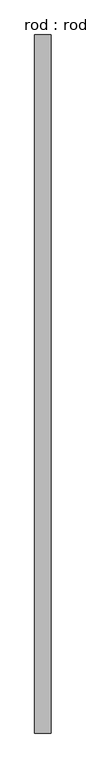
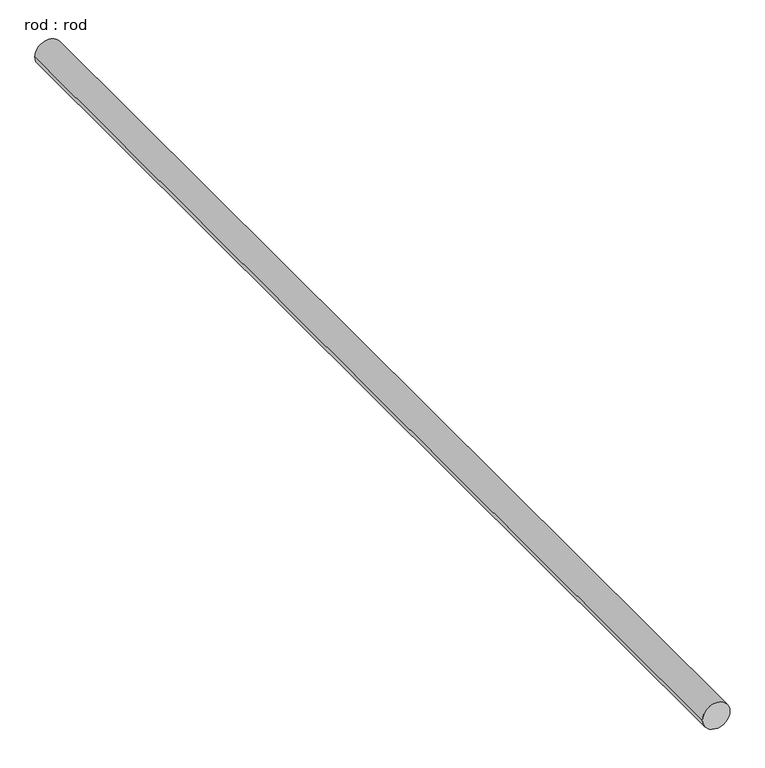
"""IFC4 building model written with IfcOpenShell, lengths in millimetres: proxy geometry, rod : rod."""

from ifc_helpers import new_model, si_unit, point, frame, frame_2d, origin, place, context, project, spatial, circle_curve, trimmed, segment, composite_curve, outline, extrude, source, transform, mapped, element, save


def rod_rod_0cf6e89c(model_context):
    return source(origin(), model_context, "Body", "SweptSolid", [
        extrude(outline(composite_curve([segment(trimmed(circle_curve(frame_2d((0.0108462, 0.0)), 200.0), [point((0.0108462, 200.0))], [point((0.0108462, -200.0))], False, "CARTESIAN"), True, "CONTINUOUS"), segment(trimmed(circle_curve(frame_2d((0.0108462, 0.0)), 200.0), [point((0.0108462, -200.0))], [point((0.0108462, 200.0))], False, "CARTESIAN"), True, "CONTINUOUS")], self_intersect=False)), frame((0.0, -4349.5154804, 0.0), z_axis=(0.0, 1.0, 0.0), x_axis=(0.0, 0.0, 1.0)), (0.0, 0.0, 1.0), 16884.4881914),
    ])


if __name__ == "__main__":
    model = new_model("IFC4")
    model_context = context("Model", 3, world=origin())
    ifc_project = project(units=[si_unit("LENGTHUNIT", "METRE", prefix="MILLI")], contexts=[model_context])
    site = spatial("IfcSite", under=ifc_project)
    building = spatial("IfcBuilding", under=site)
    placement = place(None, origin())
    rod_rod_shape = rod_rod_0cf6e89c(model_context)
    element("IfcBuildingElementProxy", 1, Name="rod : rod", ObjectType="rod : rod", at=placement, inside=building, context=model_context, shape_type="MappedRepresentation", body=[
        mapped(rod_rod_shape, transform((0.0, 0.0, 0.0), x_axis=(1.0, 0.0, 0.0), y_axis=(0.0, 1.0, 0.0), z_axis=(0.0, 0.0, 1.0))),
    ])
    save(model, "model.ifc")

# Revit data of these elements
# Type "rod : rod"
#   Default Elevation = 0
